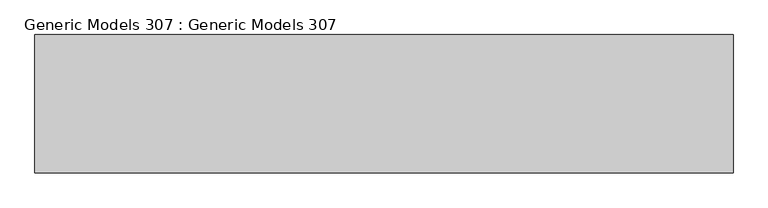
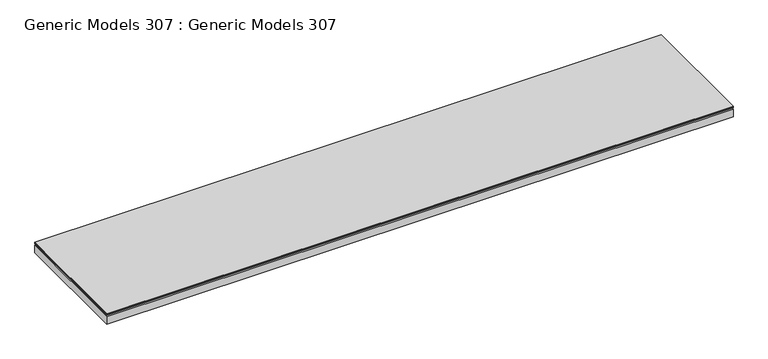
"""IFC4 building model written with IfcOpenShell, lengths in millimetres: proxy geometry, Generic Models 307 : Generic Models 307."""

from ifc_helpers import new_model, si_unit, frame, origin, place, context, project, spatial, polyline, outline, extrude, source, transform, mapped, element, save


def generic_models_307_generic_models_307_15d73da8(model_context):
    return source(origin(), model_context, "Body", "SweptSolid", [
        extrude(outline(polyline([(4057.4763704, 704.5309662), (5594.1763704, 704.5309662), (5594.1763704, 399.7309662), (4057.4763704, 399.7309662), (4057.4763704, 704.5309662)])), frame((0.0, 0.0, 129559.1462723), z_axis=(0.0, 0.0, 1.0), x_axis=(1.0, 0.0, 0.0)), (0.0, 0.0, 1.0), 1.2587721),
        extrude(outline(polyline([(4057.4763704, 704.5309662), (5594.1763704, 704.5309662), (5594.1763704, 399.7309662), (4057.4763704, 399.7309662), (4057.4763704, 704.5309662)])), frame((0.0, 0.0, 129556.3283106), z_axis=(0.0, 0.0, 1.0), x_axis=(1.0, 0.0, 0.0)), (0.0, 0.0, 1.0), 1.2587721),
        extrude(outline(polyline([(4057.4763704, 704.5309662), (5594.1763704, 704.5309662), (5594.1763704, 399.7309662), (4057.4763704, 399.7309662), (4057.4763704, 704.5309662)])), frame((0.0, 0.0, 129533.396), z_axis=(0.0, 0.0, 1.0), x_axis=(1.0, 0.0, 0.0)), (0.0, 0.0, 1.0), 19.05),
    ])


if __name__ == "__main__":
    model = new_model("IFC4")
    model_context = context("Model", 3, world=origin())
    ifc_project = project(units=[si_unit("LENGTHUNIT", "METRE", prefix="MILLI")], contexts=[model_context])
    site = spatial("IfcSite", under=ifc_project)
    building = spatial("IfcBuilding", under=site)
    placement = place(None, origin())
    generic_models_307_generic_models_307_shape = generic_models_307_generic_models_307_15d73da8(model_context)
    element("IfcBuildingElementProxy", 1, Name="Generic Models 307 : Generic Models 307", ObjectType="Generic Models 307 : Generic Models 307", at=placement, inside=building, context=model_context, shape_type="MappedRepresentation", body=[
        mapped(generic_models_307_generic_models_307_shape, transform((0.0, 0.0, 0.0), x_axis=(1.0, 0.0, 0.0), y_axis=(0.0, 1.0, 0.0), z_axis=(0.0, 0.0, 1.0))),
    ])
    save(model, "model.ifc")

# Revit data of these elements
# Element 1 (IfcBuildingElementProxy, "Generic Models 307 : Generic Models 307")
#   Materials on its faces: "_(2) LAYERS NO. 30 ASTM D226 ASPHALT SATURATED ORGANIC FELT @ ROOF", "_CDX PLYWOOD - SEE STRUCT DWGs"
# Materials
#   "_(2) LAYERS NO. 30 ASTM D226 ASPHALT SATURATED ORGANIC FELT @ ROOF": class "Generic", colour RGB 67 154 161, transparency 0, Cost = 0
#   "_CDX PLYWOOD - SEE STRUCT DWGs": class "Generic", colour RGB 98 75 74, transparency 0, Cost = 0
